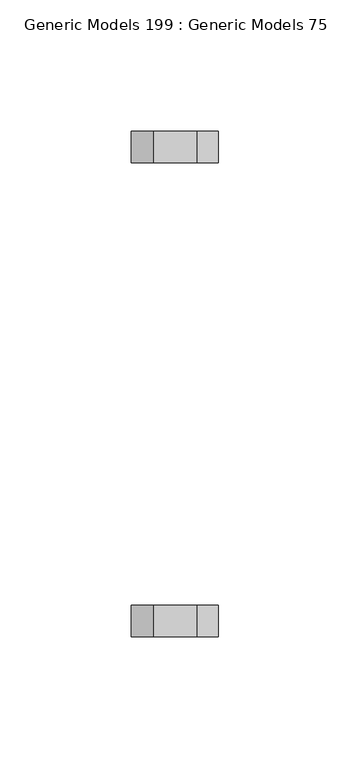
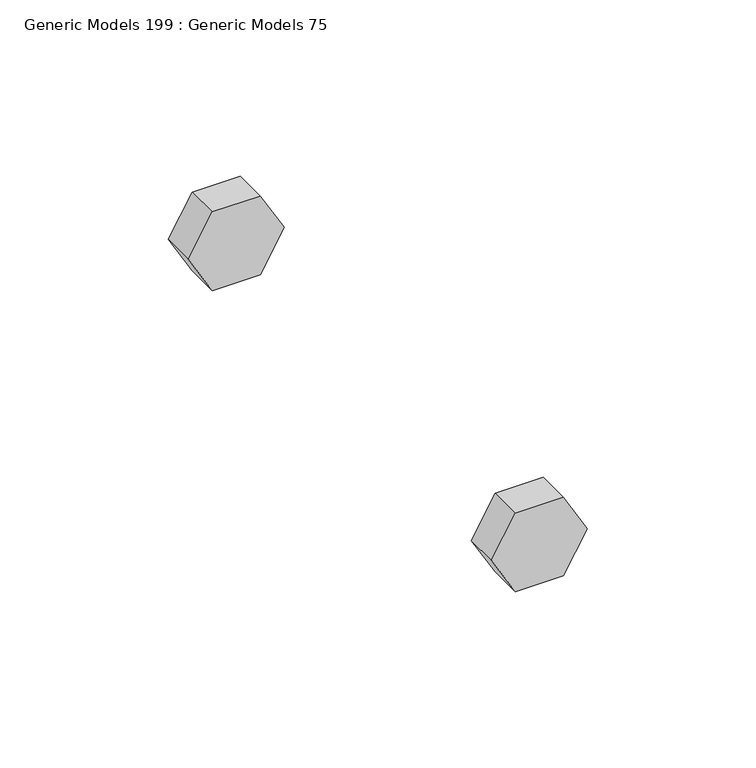
"""IFC4 building model written with IfcOpenShell, lengths in millimetres: proxy geometry, Generic Models 199 : Generic Models 75."""

from ifc_helpers import new_model, si_unit, frame, origin, place, context, project, spatial, polyline, outline, extrude, source, transform, mapped, element, save


def generic_models_199_generic_models_75_efedec74(model_context):
    return source(origin(), model_context, "Body", "SweptSolid", [
        extrude(outline(polyline([(271581.5625, 31978.2851858), (271581.5625, 31994.7829698), (271595.85, 32003.0318618), (271610.1375, 31994.7829698), (271610.1375, 31978.2851858), (271595.85, 31970.0362939), (271581.5625, 31978.2851858)])), frame((0.0, 30678.2969112, 0.0), z_axis=(0.0, 1.0, 0.0), x_axis=(0.0, 0.0, 1.0)), (0.0, 0.0, 1.0), 11.90625),
        extrude(outline(polyline([(271581.5625, 31978.2851858), (271581.5625, 31994.7829698), (271595.85, 32003.0318618), (271610.1375, 31994.7829698), (271610.1375, 31978.2851858), (271595.85, 31970.0362939), (271581.5625, 31978.2851858)])), frame((0.0, 30858.4781612, 0.0), z_axis=(0.0, 1.0, 0.0), x_axis=(0.0, 0.0, 1.0)), (0.0, 0.0, 1.0), 11.90625),
    ])


if __name__ == "__main__":
    model = new_model("IFC4")
    model_context = context("Model", 3, world=origin())
    ifc_project = project(units=[si_unit("LENGTHUNIT", "METRE", prefix="MILLI")], contexts=[model_context])
    site = spatial("IfcSite", under=ifc_project)
    building = spatial("IfcBuilding", under=site)
    placement = place(None, origin())
    generic_models_199_generic_models_75_shape = generic_models_199_generic_models_75_efedec74(model_context)
    element("IfcBuildingElementProxy", 1, Name="Generic Models 199 : Generic Models 75", ObjectType="Generic Models 199 : Generic Models 75", at=placement, inside=building, context=model_context, shape_type="MappedRepresentation", body=[
        mapped(generic_models_199_generic_models_75_shape, transform((0.0, 0.0, 0.0), x_axis=(1.0, 0.0, 0.0), y_axis=(0.0, 1.0, 0.0), z_axis=(0.0, 0.0, 1.0))),
    ])
    save(model, "model.ifc")

# Revit data of these elements
# Element 1 (IfcBuildingElementProxy, "Generic Models 199 : Generic Models 75")
#   Materials on its faces: "3/4\" GALV. THRU BOLTS"
# Materials
#   "3/4\" GALV. THRU BOLTS": class "Generic", colour RGB 105 69 171, transparency 0, Cost = 0
